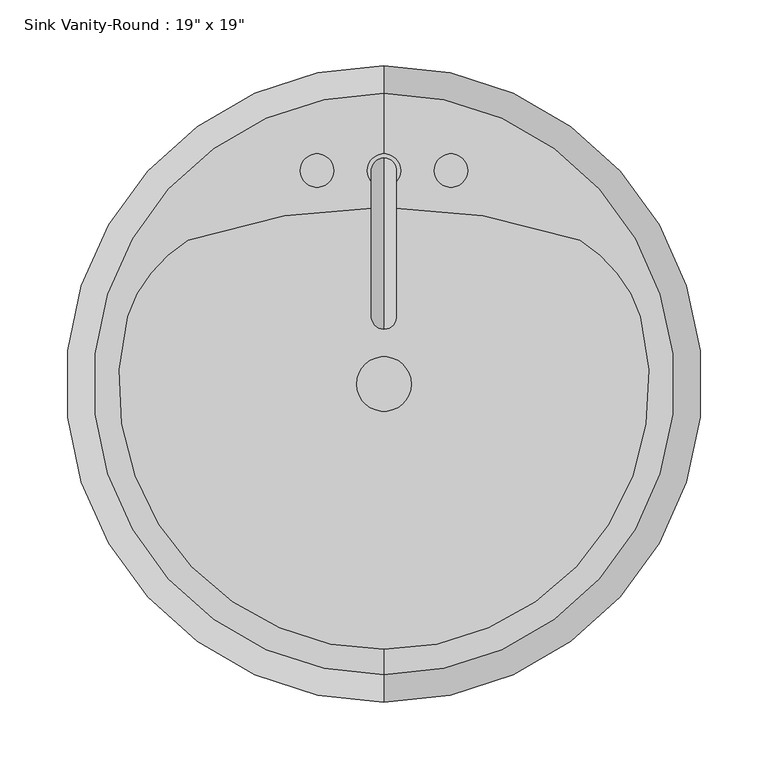
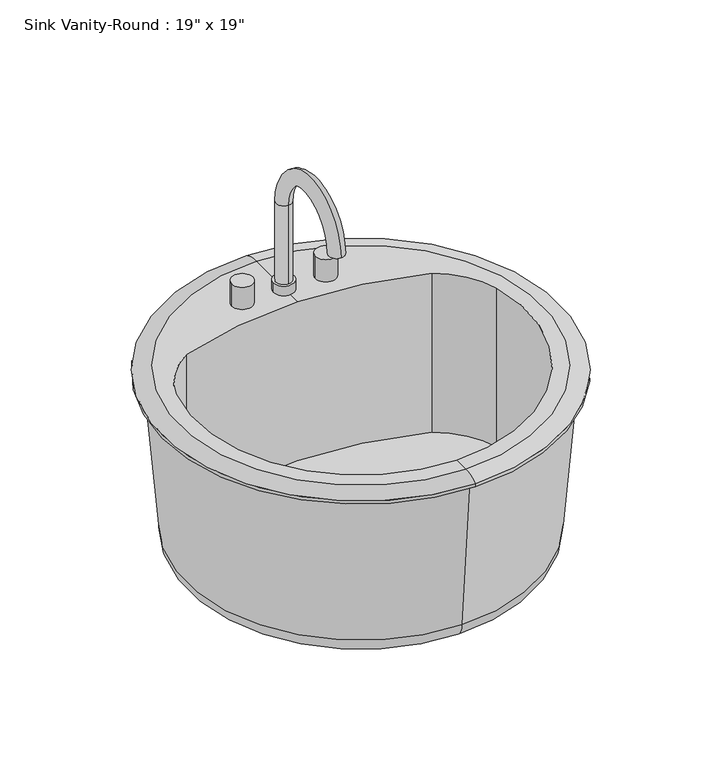
"""IFC4 building model written with IfcOpenShell, lengths in millimetres: flow terminal geometry."""

import ifcopenshell
import ifcopenshell.guid

model = None  # the IFC model being written
_history = None  # IfcOwnerHistory: only IFC2X3 demands one
_inside = {}  # id of a spatial element -> (the spatial element, [elements in it])
_under = {}  # id of a project, library or spatial element -> (it, [spatial elements below it])
_declared = {}  # id of a project -> (the project, [libraries it declares])
_typed = {}  # id of a type object -> (the type object, [elements of that type])
_made_of = {}  # id of a material, layer set ... -> (it, [elements and type objects made of it])


def new_model(schema):
    """Start an empty IFC model of exactly this schema.

    Asked for "IFC4X3", IfcOpenShell would pick the latest addendum, in which some entities
    have other attributes; the version numbers below select the first issue.
    IFC2X3 requires an IfcOwnerHistory on every rooted entity: one is made here for all.
    """
    global model, _history
    if schema == "IFC4X3":
        model = ifcopenshell.file(schema_version=(4, 3, 0, 0))
    else:
        model = ifcopenshell.file(schema=schema)
    _inside.clear()
    _under.clear()
    _declared.clear()
    _typed.clear()
    _made_of.clear()
    _history = None
    if model.schema == "IFC2X3":
        org = make("IfcOrganization", Name="unknown")
        user = make(
            "IfcPersonAndOrganization",
            ThePerson=make("IfcPerson", FamilyName="unknown"),
            TheOrganization=org,
        )
        app = make(
            "IfcApplication",
            ApplicationDeveloper=org,
            Version="unknown",
            ApplicationFullName="unknown",
            ApplicationIdentifier="unknown",
        )
        _history = make(
            "IfcOwnerHistory",
            OwningUser=user,
            OwningApplication=app,
            ChangeAction="ADDED",
            CreationDate=0,
        )
    return model


def make(cls, **values):
    """One entity of the class cls with the attributes given. An attribute that is None is left unset."""
    return model.create_entity(
        cls, **{name: value for name, value in values.items() if value is not None}
    )


def rooted(cls, **values):
    """An entity with a GlobalId (a new one), such as an element, a storey or a relation."""
    return make(cls, GlobalId=ifcopenshell.guid.new(), OwnerHistory=_history, **values)


def si_unit(unit_type, name, prefix=None):
    """IfcSIUnit, for example si_unit("LENGTHUNIT", "METRE", prefix="MILLI")."""
    return make("IfcSIUnit", UnitType=unit_type, Prefix=prefix, Name=name)


def assignment(units):
    """IfcUnitAssignment: the units of a project."""
    return None if units is None else make("IfcUnitAssignment", Units=units)


def point(xyz):
    """IfcCartesianPoint."""
    return None if xyz is None else make("IfcCartesianPoint", Coordinates=xyz)


def direction(xyz):
    """IfcDirection."""
    return None if xyz is None else make("IfcDirection", DirectionRatios=xyz)


def frame(location, z_axis=None, x_axis=None):
    """IfcAxis2Placement3D, a coordinate frame: its origin and axes. An axis left out is left unset."""
    return make(
        "IfcAxis2Placement3D",
        Location=point(location),
        Axis=direction(z_axis),
        RefDirection=direction(x_axis),
    )


def frame_2d(location, x_axis=None):
    """IfcAxis2Placement2D, a coordinate frame in the plane: its origin and x axis."""
    return make(
        "IfcAxis2Placement2D", Location=point(location), RefDirection=direction(x_axis)
    )


def origin():
    """The frame at (0, 0, 0) with its axes left unset."""
    return frame((0.0, 0.0, 0.0))


def place(relative_to, where):
    """IfcLocalPlacement: puts the frame where relative to a parent placement (None: the world)."""
    return make(
        "IfcLocalPlacement", PlacementRelTo=relative_to, RelativePlacement=where
    )


def context(
    kind, dimensions, precision=None, world=None, true_north=None, identifier=None
):
    """IfcGeometricRepresentationContext, for example the 3D "Model" context."""
    return make(
        "IfcGeometricRepresentationContext",
        ContextIdentifier=identifier,
        ContextType=kind,
        CoordinateSpaceDimension=dimensions,
        Precision=precision,
        WorldCoordinateSystem=world,
        TrueNorth=true_north,
    )


def project(units=None, contexts=None):
    """IfcProject with its units and contexts."""
    return rooted(
        "IfcProject",
        Name="project",
        RepresentationContexts=contexts,
        UnitsInContext=assignment(units),
    )


def spatial(cls, under=None, at=None, **own):
    """A site, building, storey or space (cls), placed at a placement, below another one or the project."""
    s = rooted(cls, ObjectPlacement=at, **own)
    if under is not None:
        _under.setdefault(under.id(), (under, []))[1].append(s)
    return s


def polyline(points):
    """IfcPolyline through the points."""
    return make("IfcPolyline", Points=[point(p) for p in points])


def circle_curve(where, radius):
    """IfcCircle in the frame where."""
    return make("IfcCircle", Position=where, Radius=radius)


def ellipse_curve(where, semi_axis1, semi_axis2):
    """IfcEllipse in the frame where."""
    return make(
        "IfcEllipse", Position=where, SemiAxis1=semi_axis1, SemiAxis2=semi_axis2
    )


def trimmed(basis, trim1, trim2, sense, master):
    """IfcTrimmedCurve: the piece of a basis curve between two trims."""
    return make(
        "IfcTrimmedCurve",
        BasisCurve=basis,
        Trim1=trim1,
        Trim2=trim2,
        SenseAgreement=sense,
        MasterRepresentation=master,
    )


def segment(curve, same_sense, transition):
    """IfcCompositeCurveSegment."""
    return make(
        "IfcCompositeCurveSegment",
        Transition=transition,
        SameSense=same_sense,
        ParentCurve=curve,
    )


def composite_curve(segments, self_intersect=None):
    """IfcCompositeCurve: segments joined end to end."""
    return make("IfcCompositeCurve", Segments=segments, SelfIntersect=self_intersect)


def outline(outer, holes=None, kind="AREA"):
    """IfcArbitraryClosedProfileDef: a profile drawn as a closed curve; with holes, ...WithVoids."""
    if holes is None:
        return make("IfcArbitraryClosedProfileDef", ProfileType=kind, OuterCurve=outer)
    return make(
        "IfcArbitraryProfileDefWithVoids",
        ProfileType=kind,
        OuterCurve=outer,
        InnerCurves=holes,
    )


def extrude(swept, where, along, depth):
    """IfcExtrudedAreaSolid: the profile swept, set in the frame where, extruded along a direction by depth."""
    return make(
        "IfcExtrudedAreaSolid",
        SweptArea=swept,
        Position=where,
        ExtrudedDirection=direction(along),
        Depth=depth,
    )


def shape(context_of_items, identifier, shape_type, items):
    """IfcShapeRepresentation: the items that make up one representation, for example the "Body"."""
    return make(
        "IfcShapeRepresentation",
        ContextOfItems=context_of_items,
        RepresentationIdentifier=identifier,
        RepresentationType=shape_type,
        Items=items,
    )


def source(mapping_origin, context_of_items, identifier, shape_type, items):
    """IfcRepresentationMap: a shape defined once, which mapped items show again and again."""
    return make(
        "IfcRepresentationMap",
        MappingOrigin=mapping_origin,
        MappedRepresentation=shape(context_of_items, identifier, shape_type, items),
    )


def transform(
    local_origin,
    x_axis=None,
    y_axis=None,
    z_axis=None,
    scale=None,
    scale2=None,
    scale3=None,
    uniform=True,
):
    """IfcCartesianTransformationOperator3D, or its non-uniform kind. x_axis, y_axis, z_axis: its Axis1, 2, 3."""
    if uniform:
        return make(
            "IfcCartesianTransformationOperator3D",
            Axis1=direction(x_axis),
            Axis2=direction(y_axis),
            LocalOrigin=point(local_origin),
            Scale=scale,
            Axis3=direction(z_axis),
        )
    return make(
        "IfcCartesianTransformationOperator3DnonUniform",
        Axis1=direction(x_axis),
        Axis2=direction(y_axis),
        LocalOrigin=point(local_origin),
        Scale=scale,
        Axis3=direction(z_axis),
        Scale2=scale2,
        Scale3=scale3,
    )


def mapped(mapping_source, mapping_target):
    """IfcMappedItem: shows the shape of a source again, moved by a transform."""
    return make(
        "IfcMappedItem", MappingSource=mapping_source, MappingTarget=mapping_target
    )


def made_of(thing, what):
    """Note that an element or type object is made of a material, layer set ...; save() writes the relation."""
    if what is not None:
        _made_of.setdefault(what.id(), (what, []))[1].append(thing)
    return thing


def element(
    cls,
    number,
    at=None,
    inside=None,
    cuts=None,
    type_object=None,
    material=None,
    context=None,
    identifier="Body",
    shape_type=None,
    held_by="IfcProductDefinitionShape",
    body=None,
    shapes=None,
    **own,
):
    """One element of the class cls, such as IfcWall. Its Tag is "e" and its number.

    at: its placement. inside: the storey or other place that contains it. cuts: it is an
    opening in that element (IfcRelVoidsElement). A single representation is given by context,
    identifier, shape_type and body (its items); several are given by shapes. held_by: the class
    of the entity that holds the representations. save() writes the other relations.
    """
    e = rooted(cls, Tag="e%d" % number, ObjectPlacement=at, **own)
    if body is not None:
        shapes = [shape(context, identifier, shape_type, body)]
    if shapes is not None:
        e.Representation = make(held_by, Representations=shapes)
    if inside is not None:
        _inside.setdefault(inside.id(), (inside, []))[1].append(e)
    if cuts is not None:
        rooted(
            "IfcRelVoidsElement", RelatingBuildingElement=cuts, RelatedOpeningElement=e
        )
    if type_object is not None:
        _typed.setdefault(type_object.id(), (type_object, []))[1].append(e)
    return made_of(e, material)


def aggregate(whole, parts):
    """IfcRelAggregates: a whole, such as a stair, and the parts it consists of."""
    return rooted("IfcRelAggregates", RelatingObject=whole, RelatedObjects=parts)


def save(model, path):
    """Write the relations noted so far, then the file.

    IfcRelAggregates (storeys below a building ...), IfcRelContainedInSpatialStructure (elements
    in a storey), IfcRelDefinesByType, IfcRelAssociatesMaterial and IfcRelDeclares: one each for
    every whole, place, type object, material and project.
    """
    for whole, parts in _under.values():
        aggregate(whole, parts)
    for where, things in _inside.values():
        rooted(
            "IfcRelContainedInSpatialStructure",
            RelatedElements=things,
            RelatingStructure=where,
        )
    for kind, things in _typed.values():
        rooted("IfcRelDefinesByType", RelatedObjects=things, RelatingType=kind)
    for what, things in _made_of.values():
        rooted("IfcRelAssociatesMaterial", RelatedObjects=things, RelatingMaterial=what)
    for by, libraries in _declared.values():
        rooted("IfcRelDeclares", RelatingContext=by, RelatedDefinitions=libraries)
    model.write(path)


def plane_surface(at):
    """IfcPlane: the flat surface through the origin of the frame at, square to its z axis."""
    return make("IfcPlane", Position=at)


def cylinder_surface(at, radius):
    """IfcCylindricalSurface: all points at the distance radius from the z axis of the frame at."""
    return make("IfcCylindricalSurface", Position=at, Radius=radius)


def revolved_surface(curve, axis_point, axis_direction):
    """IfcSurfaceOfRevolution: the curve turned about the line through axis_point along axis_direction."""
    return make(
        "IfcSurfaceOfRevolution",
        SweptCurve=make("IfcArbitraryOpenProfileDef", ProfileType="CURVE", Curve=curve),
        AxisPosition=make("IfcAxis1Placement", Location=point(axis_point), Axis=direction(axis_direction)),
    )


def advanced_brep(points, edges, surfaces, faces):
    """IfcAdvancedBrep: a solid bounded by faces that lie on surfaces and meet in shared edges.

    An edge is (start, end): straight between two places in points (the first is 0);
    or (start, end, curve); or (start, end, curve, False) where it runs against its curve.
    A face is (place in surfaces, loops), or (place, loops, False) where it looks against
    its surface's normal. A loop lists edges by number (the first is 1), with a minus sign
    where the edge is run from its end to its start. The first loop is the outer one.
    """
    corners = [point(p) for p in points]
    vertices = [make("IfcVertexPoint", VertexGeometry=c) for c in corners]
    made = []
    for start, end, *more in edges:
        made.append(
            make(
                "IfcEdgeCurve",
                EdgeStart=vertices[start],
                EdgeEnd=vertices[end],
                EdgeGeometry=more[0] if more else make("IfcPolyline", Points=[corners[start], corners[end]]),
                SameSense=more[1] if len(more) > 1 else True,
            )
        )
    hull = []
    for where, loops, *sense in faces:
        bounds = []
        for j, loop in enumerate(loops):
            ring = [make("IfcOrientedEdge", EdgeElement=made[abs(k) - 1], Orientation=k > 0) for k in loop]
            bounds.append(
                make(
                    "IfcFaceOuterBound" if j == 0 else "IfcFaceBound",
                    Bound=make("IfcEdgeLoop", EdgeList=ring),
                    Orientation=True,
                )
            )
        hull.append(make("IfcAdvancedFace", Bounds=bounds, FaceSurface=surfaces[where], SameSense=sense[0] if sense else True))
    return make("IfcAdvancedBrep", Outer=make("IfcClosedShell", CfsFaces=hull))


def flow_terminal_5184717d(model_context):
    return source(origin(), model_context, "Body", "SolidModel", [
        advanced_brep(
        [(96.6517406, 237.5677185, 796.925), (96.6517406, 256.6177185, 796.925), (96.6517406, 237.5677185, 909.6375), (96.6517406, 256.6177185, 909.6375), (96.6517406, 145.7775038, 909.6375), (96.6517406, 126.7275038, 909.6375)],
        [
            (0, 1, circle_curve(frame((96.6517406, 247.0927185, 796.925), z_axis=(0.0, 0.0, -1.0), x_axis=(0.0, 1.0, 0.0)), 9.525)),
            (1, 0, circle_curve(frame((96.6517406, 247.0927185, 796.925), z_axis=(0.0, 0.0, -1.0), x_axis=(0.0, 1.0, 0.0)), 9.525)),
            (0, 2),
            (2, 3, circle_curve(frame((96.6517406, 247.0927185, 909.6375), z_axis=(0.0, 0.0, -1.0), x_axis=(0.0, 1.0, 0.0)), 9.525)),
            (3, 1),
            (3, 2, circle_curve(frame((96.6517406, 247.0927185, 909.6375), z_axis=(0.0, 0.0, -1.0), x_axis=(0.0, 1.0, 0.0)), 9.525)),
            (4, 5, circle_curve(frame((96.6517406, 136.2525038, 909.6375), z_axis=(0.0, 0.0, -1.0), x_axis=(0.0, -1.0, 0.0)), 9.525)),
            (5, 4, circle_curve(frame((96.6517406, 136.2525038, 909.6375), z_axis=(0.0, 0.0, -1.0), x_axis=(0.0, -1.0, 0.0)), 9.525)),
            (5, 3, circle_curve(frame((96.6517406, 191.6726112, 909.6375), z_axis=(-1.0, 0.0, 0.0), x_axis=(0.0, 1.0, 0.0)), 64.9451073)),
            (2, 4, circle_curve(frame((96.6517406, 191.6726112, 909.6375), z_axis=(1.0, 0.0, 0.0), x_axis=(0.0, 1.0, 0.0)), 45.8951073)),
        ],
        [
            plane_surface(frame((96.6517406, 237.5677185, 796.925), z_axis=(0.0, 0.0, -1.0), x_axis=(1.0, 0.0, 0.0))),
            cylinder_surface(frame((96.6517406, 247.0927185, 796.925), z_axis=(0.0, 0.0, -1.0), x_axis=(0.0, 1.0, 0.0)), 9.525),
            plane_surface(frame((96.6517406, 191.6726112, 909.6375), z_axis=(0.0, 0.0, -1.0), x_axis=(0.0, -1.0, 0.0))),
            revolved_surface(trimmed(ellipse_curve(frame((96.6517406, 247.0927185, 909.6375), z_axis=(0.0, 0.0, -1.0), x_axis=(0.0, 1.0, 0.0)), 9.525, 9.525), [point((96.6517406, 237.5677185, 909.6375))], [point((96.6517406, 256.6177185, 909.6375))], True, "CARTESIAN"), (96.6517406, 191.6726112, 909.6375), (1.0, 0.0, 0.0)),
            revolved_surface(trimmed(ellipse_curve(frame((96.6517406, 247.0927185, 909.6375), z_axis=(0.0, 0.0, -1.0), x_axis=(0.0, 1.0, 0.0)), 9.525, 9.525), [point((96.6517406, 256.6177185, 909.6375))], [point((96.6517406, 237.5677185, 909.6375))], True, "CARTESIAN"), (96.6517406, 191.6726112, 909.6375), (1.0, 0.0, 0.0)),
        ],
        [
            (0, [[1, 2]]),
            (1, [[-1, 3, 4, 5]]),
            (1, [[-2, -5, 6, -3]]),
            (2, [[7, 8]]),
            (3, [[9, -4, 10, -8]]),
            (4, [[-10, -6, -9, -7]]),
        ],
    ),
        extrude(outline(composite_curve([segment(trimmed(circle_curve(frame_2d((96.6517406, 247.0927185)), 12.7), [point((83.9517406, 247.0927185))], [point((109.3517406, 247.0927185))], False, "CARTESIAN"), True, "CONTINUOUS"), segment(trimmed(circle_curve(frame_2d((96.6517406, 247.0927185)), 12.7), [point((109.3517406, 247.0927185))], [point((83.9517406, 247.0927185))], False, "CARTESIAN"), True, "CONTINUOUS")], self_intersect=False)), frame((0.0, 0.0, 796.925), z_axis=(0.0, 0.0, 1.0), x_axis=(1.0, 0.0, 0.0)), (0.0, 0.0, 1.0), 12.2352909),
        extrude(outline(composite_curve([segment(trimmed(circle_curve(frame_2d((45.8517406, 247.0927185)), 12.7), [point((33.1517406, 247.0927185))], [point((58.5517406, 247.0927185))], False, "CARTESIAN"), True, "CONTINUOUS"), segment(trimmed(circle_curve(frame_2d((45.8517406, 247.0927185)), 12.7), [point((58.5517406, 247.0927185))], [point((33.1517406, 247.0927185))], False, "CARTESIAN"), True, "CONTINUOUS")], self_intersect=False)), frame((0.0, 0.0, 796.925), z_axis=(0.0, 0.0, 1.0), x_axis=(1.0, 0.0, 0.0)), (0.0, 0.0, 1.0), 28.575),
        extrude(outline(composite_curve([segment(trimmed(circle_curve(frame_2d((147.4517406, 247.0927185)), 12.7), [point((134.7517406, 247.0927185))], [point((160.1517406, 247.0927185))], False, "CARTESIAN"), True, "CONTINUOUS"), segment(trimmed(circle_curve(frame_2d((147.4517406, 247.0927185)), 12.7), [point((160.1517406, 247.0927185))], [point((134.7517406, 247.0927185))], False, "CARTESIAN"), True, "CONTINUOUS")], self_intersect=False)), frame((0.0, 0.0, 796.925), z_axis=(0.0, 0.0, 1.0), x_axis=(1.0, 0.0, 0.0)), (0.0, 0.0, 1.0), 28.575),
        extrude(outline(composite_curve([segment(trimmed(circle_curve(frame_2d((96.6517406, 85.1677185)), 20.6375), [point((76.0142406, 85.1677185))], [point((117.2892406, 85.1677185))], False, "CARTESIAN"), True, "CONTINUOUS"), segment(trimmed(circle_curve(frame_2d((96.6517406, 85.1677185)), 20.6375), [point((117.2892406, 85.1677185))], [point((76.0142406, 85.1677185))], False, "CARTESIAN"), True, "CONTINUOUS")], self_intersect=False)), frame((0.0, 0.0, 571.5), z_axis=(0.0, 0.0, 1.0), x_axis=(1.0, 0.0, 0.0)), (0.0, 0.0, 1.0), 21.1842611),
        advanced_brep(
        [(96.6517406, -135.3870093, 796.925), (96.6517406, 305.7224463, 796.925), (96.6517406, 326.4677185, 791.36875), (96.6517406, -156.1322815, 791.36875), (96.6517406, -116.2405705, 796.925), (-98.1703414, 136.2525038, 796.925), (-52.1534933, 194.0861398, 796.925), (96.6517406, 219.2662048, 796.925), (245.4569744, 194.0861398, 796.925), (291.4738225, 136.2525038, 796.925), (96.6517406, -107.1264028, 571.5), (96.6517406, 277.4618398, 571.5), (96.6517406, 85.1677185, 571.5), (96.6517406, -127.6827361, 592.6842611), (96.6517406, 298.0181731, 592.6842611), (96.6517406, -144.2260315, 787.4), (96.6517406, 314.5614685, 787.4), (96.6517406, -156.1322815, 787.4), (96.6517406, 326.4677185, 787.4), (245.4569744, 194.0861398, 592.6842611), (-52.1534933, 194.0861398, 592.6842611), (-98.1703414, 136.2525038, 592.6842611), (291.4738225, 136.2525038, 592.6842611)],
        [
            (0, 1, circle_curve(frame((96.6517406, 85.1677185, 796.925), z_axis=(0.0, 0.0, -1.0), x_axis=(0.0, 1.0, 0.0)), 220.5547278)),
            (1, 2, circle_curve(frame((96.6517406, 309.4374616, 769.289434), z_axis=(-1.0, 0.0, 0.0), x_axis=(0.0, 1.0, 0.0)), 27.8841505)),
            (2, 3, circle_curve(frame((96.6517406, 85.1677185, 791.36875), z_axis=(0.0, 0.0, 1.0), x_axis=(0.0, 1.0, 0.0)), 241.3)),
            (3, 0, circle_curve(frame((96.6517406, -139.1020246, 769.289434), z_axis=(-1.0, 0.0, 0.0), x_axis=(0.0, -1.0, 0.0)), 27.8841505)),
            (1, 0, circle_curve(frame((96.6517406, 85.1677185, 796.925), z_axis=(0.0, 0.0, -1.0), x_axis=(0.0, 1.0, 0.0)), 220.5547278)),
            (3, 2, circle_curve(frame((96.6517406, 85.1677185, 791.36875), z_axis=(0.0, 0.0, 1.0), x_axis=(0.0, 1.0, 0.0)), 241.3)),
            (0, 4),
            (4, 5, circle_curve(frame((96.6517406, 85.1677185, 796.925), z_axis=(0.0, 0.0, -1.0), x_axis=(1.0, 0.0, 0.0)), 201.408289)),
            (5, 6, circle_curve(frame((1.3689689, 104.2755165, 796.925), z_axis=(0.0, 0.0, -1.0), x_axis=(1.0, 0.0, 0.0)), 104.5495194)),
            (6, 7, circle_curve(frame((96.6517406, -233.0168462, 796.925), z_axis=(0.0, 0.0, -1.0), x_axis=(1.0, 0.0, 0.0)), 452.283051)),
            (7, 1),
            (7, 8, circle_curve(frame((96.6517406, -233.0168462, 796.925), z_axis=(0.0, 0.0, -1.0), x_axis=(1.0, 0.0, 0.0)), 452.283051)),
            (8, 9, circle_curve(frame((191.9345122, 104.2755165, 796.925), z_axis=(0.0, 0.0, -1.0), x_axis=(1.0, 0.0, 0.0)), 104.5495194)),
            (9, 4, circle_curve(frame((96.6517406, 85.1677185, 796.925), z_axis=(0.0, 0.0, -1.0), x_axis=(1.0, 0.0, 0.0)), 201.408289)),
            (10, 11, circle_curve(frame((96.6517406, 85.1677185, 571.5), z_axis=(0.0, 0.0, -1.0), x_axis=(0.0, 1.0, 0.0)), 192.2941213)),
            (11, 12),
            (12, 10),
            (11, 10, circle_curve(frame((96.6517406, 85.1677185, 571.5), z_axis=(0.0, 0.0, -1.0), x_axis=(0.0, 1.0, 0.0)), 192.2941213)),
            (10, 13, circle_curve(frame((96.6517406, -107.1264028, 592.0656396), z_axis=(-1.0, 0.0, 0.0), x_axis=(0.0, -1.0, 0.0)), 20.5656396)),
            (13, 14, circle_curve(frame((96.6517406, 85.1677185, 592.6842611), z_axis=(0.0, 0.0, -1.0), x_axis=(0.0, 1.0, 0.0)), 212.8504546)),
            (14, 11, circle_curve(frame((96.6517406, 277.4618398, 592.0656396), z_axis=(-1.0, 0.0, 0.0), x_axis=(0.0, 1.0, 0.0)), 20.5656396)),
            (14, 13, circle_curve(frame((96.6517406, 85.1677185, 592.6842611), z_axis=(0.0, 0.0, -1.0), x_axis=(0.0, 1.0, 0.0)), 212.8504546)),
            (13, 15),
            (15, 16, circle_curve(frame((96.6517406, 85.1677185, 787.4), z_axis=(0.0, 0.0, -1.0), x_axis=(0.0, 1.0, 0.0)), 229.39375)),
            (16, 14),
            (16, 15, circle_curve(frame((96.6517406, 85.1677185, 787.4), z_axis=(0.0, 0.0, -1.0), x_axis=(0.0, 1.0, 0.0)), 229.39375)),
            (15, 17),
            (17, 18, circle_curve(frame((96.6517406, 85.1677185, 787.4), z_axis=(0.0, 0.0, -1.0), x_axis=(0.0, 1.0, 0.0)), 241.3)),
            (18, 16),
            (18, 17, circle_curve(frame((96.6517406, 85.1677185, 787.4), z_axis=(0.0, 0.0, -1.0), x_axis=(0.0, 1.0, 0.0)), 241.3)),
            (2, 18),
            (17, 3),
            (19, 20, circle_curve(frame((96.6517406, -233.0168462, 592.6842611), z_axis=(0.0, 0.0, 1.0), x_axis=(1.0, 0.0, 0.0)), 452.283051)),
            (20, 21, circle_curve(frame((1.3689689, 104.2755165, 592.6842611), z_axis=(0.0, 0.0, 1.0), x_axis=(1.0, 0.0, 0.0)), 104.5495194)),
            (21, 22, circle_curve(frame((96.6517406, 85.1677185, 592.6842611), z_axis=(0.0, 0.0, 1.0), x_axis=(1.0, 0.0, 0.0)), 201.408289)),
            (22, 19, circle_curve(frame((191.9345122, 104.2755165, 592.6842611), z_axis=(0.0, 0.0, 1.0), x_axis=(1.0, 0.0, 0.0)), 104.5495194)),
            (19, 8),
            (6, 20),
            (5, 21),
            (9, 22),
        ],
        [
            revolved_surface(trimmed(ellipse_curve(frame((96.6517406, 309.4374616, 769.289434), z_axis=(1.0, 0.0, 0.0), x_axis=(0.0, 1.0, 0.0)), 27.8841505, 27.8841505), [point((96.6517406, 326.4677185, 791.36875))], [point((96.6517406, 305.7224463, 796.925))], True, "CARTESIAN"), (96.6517406, 85.1677185, 796.925), (0.0, 0.0, 1.0)),
            plane_surface(frame((96.6517406, 85.1677185, 796.925), z_axis=(0.0, 0.0, 1.0), x_axis=(0.0, 1.0, 0.0))),
            plane_surface(frame((96.6517406, 85.1677185, 571.5), z_axis=(0.0, 0.0, -1.0), x_axis=(0.0, 1.0, 0.0))),
            revolved_surface(trimmed(ellipse_curve(frame((96.6517406, 277.4618398, 592.0656396), z_axis=(1.0, 0.0, 0.0), x_axis=(0.0, 1.0, 0.0)), 20.5656396, 20.5656396), [point((96.6517406, 277.4618398, 571.5))], [point((96.6517406, 298.0181731, 592.6842611))], True, "CARTESIAN"), (96.6517406, 85.1677185, 796.925), (0.0, 0.0, 1.0)),
            revolved_surface(polyline([(96.6517406, 298.0181731, 592.6842611), (96.6517406, 314.5614685, 787.4)]), (96.6517406, 85.1677185, 796.925), (0.0, 0.0, 1.0)),
            plane_surface(frame((96.6517406, 85.1677185, 787.4), z_axis=(0.0, 0.0, -1.0), x_axis=(0.0, 1.0, 0.0))),
            cylinder_surface(frame((96.6517406, 85.1677185, 796.925), z_axis=(0.0, 0.0, 1.0), x_axis=(0.0, 1.0, 0.0)), 241.3),
            plane_surface(frame((548.9347916, -233.0168462, 592.6842611), z_axis=(0.0, 0.0, 1.0), x_axis=(0.0, -1.0, 0.0))),
            revolved_surface(polyline([(548.9347916, -233.0168462, 796.925), (548.9347916, -233.0168462, 592.6842611)]), (96.6517406, -233.0168462, 592.6842611), (0.0, 0.0, 1.0)),
            revolved_surface(polyline([(105.91848829999999, 104.2755165, 796.925), (105.91848829999999, 104.2755165, 592.6842611)]), (1.3689689, 104.2755165, 592.6842611), (0.0, 0.0, 1.0)),
            revolved_surface(polyline([(298.0600296, 85.1677185, 796.925), (298.0600296, 85.1677185, 592.6842611)]), (96.6517406, 85.1677185, 592.6842611), (0.0, 0.0, 1.0)),
            revolved_surface(polyline([(296.4840316, 104.2755165, 796.925), (296.4840316, 104.2755165, 592.6842611)]), (191.9345122, 104.2755165, 592.6842611), (0.0, 0.0, 1.0)),
        ],
        [
            (0, [[1, 2, 3, 4]]),
            (0, [[-2, 5, -4, 6]]),
            (1, [[-1, 7, 8, 9, 10, 11]]),
            (1, [[-5, -11, 12, 13, 14, -7]]),
            (2, [[15, 16, 17]]),
            (2, [[-16, 18, -17]]),
            (3, [[-15, 19, 20, 21]]),
            (3, [[-18, -21, 22, -19]]),
            (4, [[-20, 23, 24, 25]]),
            (4, [[-22, -25, 26, -23]]),
            (5, [[-24, 27, 28, 29]]),
            (5, [[-26, -29, 30, -27]]),
            (6, [[-3, 31, -28, 32]]),
            (6, [[-6, -32, -30, -31]]),
            (7, [[33, 34, 35, 36]]),
            (8, [[-33, 37, -12, -10, 38]]),
            (9, [[-34, -38, -9, 39]]),
            (10, [[-35, -39, -8, -14, 40]]),
            (11, [[-36, -40, -13, -37]]),
        ],
    ),
    ])


if __name__ == "__main__":
    model = new_model("IFC4")
    model_context = context("Model", 3, world=origin())
    ifc_project = project(units=[si_unit("LENGTHUNIT", "METRE", prefix="MILLI")], contexts=[model_context])
    site = spatial("IfcSite", under=ifc_project)
    building = spatial("IfcBuilding", under=site)
    placement = place(None, origin())
    flow_terminal_shape = flow_terminal_5184717d(model_context)
    element("IfcFlowTerminal", 1, ObjectType="Sink Vanity-Round : 19\" x 19\"", at=placement, inside=building, context=model_context, shape_type="MappedRepresentation", body=[
        mapped(flow_terminal_shape, transform((0.0, 0.0, 0.0), x_axis=(1.0, 0.0, 0.0), y_axis=(0.0, 1.0, 0.0), z_axis=(0.0, 0.0, 1.0))),
    ])
    save(model, "model.ifc")

# Revit data of these elements
# Type "Sink Vanity-Round : 19\" x 19\""
#   Assembly Code = "D2010400"
#   Top Of Counter = 2' - 7"
#   Basin Material = Porcelain - Linen
#   Faucet Material = Metal - Steel, Polished
#   Default Elevation = 0
# Element 1 (IfcFlowTerminal, "Sink Vanity-Round : 19\" x 19\"")
#   Materials on its faces: "Porcelain - Linen", "Metal - Steel, Polished"
# Materials
#   "Porcelain - Linen": class "Unassigned", colour RGB 249 239 230, transparency 0
#   "Metal - Steel, Polished": class "Unassigned", colour RGB 57 57 57, transparency 0
